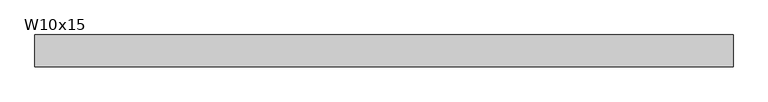
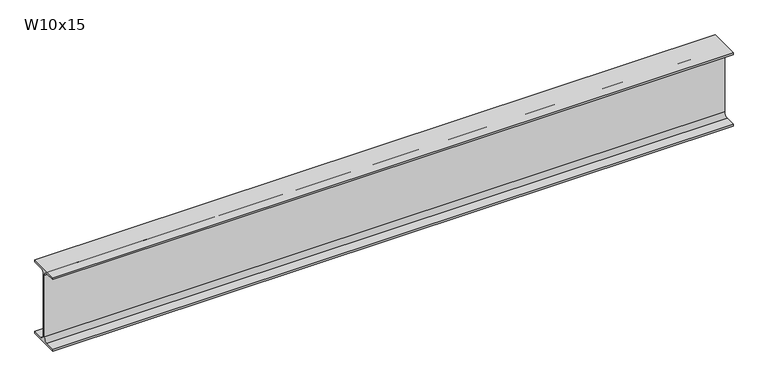
"""IFC4 building model written with IfcOpenShell, lengths in millimetres: beam geometry, RME W-Wide Flange : W10x15."""

from ifc_helpers import new_model, si_unit, point, frame, frame_2d, origin, place, context, project, spatial, polyline, circle_curve, trimmed, segment, composite_curve, outline, extrude, source, transform, mapped, element, save


def w10x15_e471eb64(model_context):
    return source(origin(), model_context, "Body", "SweptSolid", [
        extrude(outline(composite_curve([segment(polyline([(50.8, -120.142), (50.8, -127.0), (-50.8, -127.0), (-50.8, -120.142), (-16.7005, -120.142)]), True, "CONTINUOUS"), segment(trimmed(circle_curve(frame_2d((-16.7005, -106.3625)), 13.7795), [point((-16.7005, -120.142))], [point((-2.921, -106.3625))], True, "CARTESIAN"), True, "CONTINUOUS"), segment(polyline([(-2.921, -106.3625), (-2.921, 106.3625)]), True, "CONTINUOUS"), segment(trimmed(circle_curve(frame_2d((-16.7005, 106.3625)), 13.7795), [point((-2.921, 106.3625))], [point((-16.7005, 120.142))], True, "CARTESIAN"), True, "CONTINUOUS"), segment(polyline([(-16.7005, 120.142), (-50.8, 120.142), (-50.8, 127.0), (50.8, 127.0), (50.8, 120.142), (16.7005, 120.142)]), True, "CONTINUOUS"), segment(trimmed(circle_curve(frame_2d((16.7005, 106.3625)), 13.7795), [point((16.7005, 120.142))], [point((2.921, 106.3625))], True, "CARTESIAN"), True, "CONTINUOUS"), segment(polyline([(2.921, 106.3625), (2.921, -106.3625)]), True, "CONTINUOUS"), segment(trimmed(circle_curve(frame_2d((16.7005, -106.3625)), 13.7795), [point((2.921, -106.3625))], [point((16.7005, -120.142))], True, "CARTESIAN"), True, "CONTINUOUS"), segment(polyline([(16.7005, -120.142), (50.8, -120.142)]), True, "CONTINUOUS")], self_intersect=False)), frame((-1079.373, 0.0, 0.0), z_axis=(1.0, 0.0, 0.0), x_axis=(0.0, 1.0, 0.0)), (0.0, 0.0, 1.0), 2222.373),
    ])


if __name__ == "__main__":
    model = new_model("IFC4")
    model_context = context("Model", 3, world=origin())
    ifc_project = project(units=[si_unit("LENGTHUNIT", "METRE", prefix="MILLI")], contexts=[model_context])
    site = spatial("IfcSite", under=ifc_project)
    building = spatial("IfcBuilding", under=site)
    placement = place(None, origin())
    w10x15_shape = w10x15_e471eb64(model_context)
    element("IfcBeam", 1, ObjectType="RME W-Wide Flange : W10x15", at=placement, inside=building, context=model_context, shape_type="MappedRepresentation", body=[
        mapped(w10x15_shape, transform((0.0, 0.0, 0.0), x_axis=(1.0, 0.0, 0.0), y_axis=(0.0, 1.0, 0.0), z_axis=(0.0, 0.0, 1.0))),
    ])
    save(model, "model.ifc")

# Revit data of these elements
# Type "RME W-Wide Flange : W10x15"
#   WELD P [instance default] = ""
#   WELD LE [instance default] = ""
#   WELD D [instance default] = ""
#   TOP SECTION SIZE [instance default] = ""
#   TOP SECTION LENGTH [instance default] = ""
#   REMARKS [instance default] = ""
#   REINF TYPE [instance default] = ""
#   Nominal Size = "W24"
#   End Bearing Capacity [instance default] = ""
#   BOT SECTION SIZE [instance default] = ""
#   BOT SECTION LENGTH [instance default] = ""
#   Assembly Code = "B10"
#   W = 15
#   Start Extension Calculation [instance default] = 10' - 0"
#   Start Extension [instance default] = -0' - 0 1/2"
#   End Extension Calculation [instance default] = 10' - 0"
#   End Extension [instance default] = -0' - 0 1/2"
#   Length [instance default] = 5' - 0"
#   bf = 0' - 4"
#   d = 0' - 10"
#   k = 0' - 0 13/16"
#   k2 = 0' - 0.5425"
#   tf = 0' - 0.27"
#   tw = 0' - 0.23"
#   A = 0.030625 SF
#   Structural Material [instance default] = Metal - Steel - ASTM A992
# Element 1 (IfcBeam, "RME W-Wide Flange : W10x15")
#   Length = 7' - 6"
#   Materials on its faces: "Metal - Steel - ASTM A992"
# Materials
#   "Metal - Steel - ASTM A992": class "Metal", colour RGB 255 128 0, transparency 0
